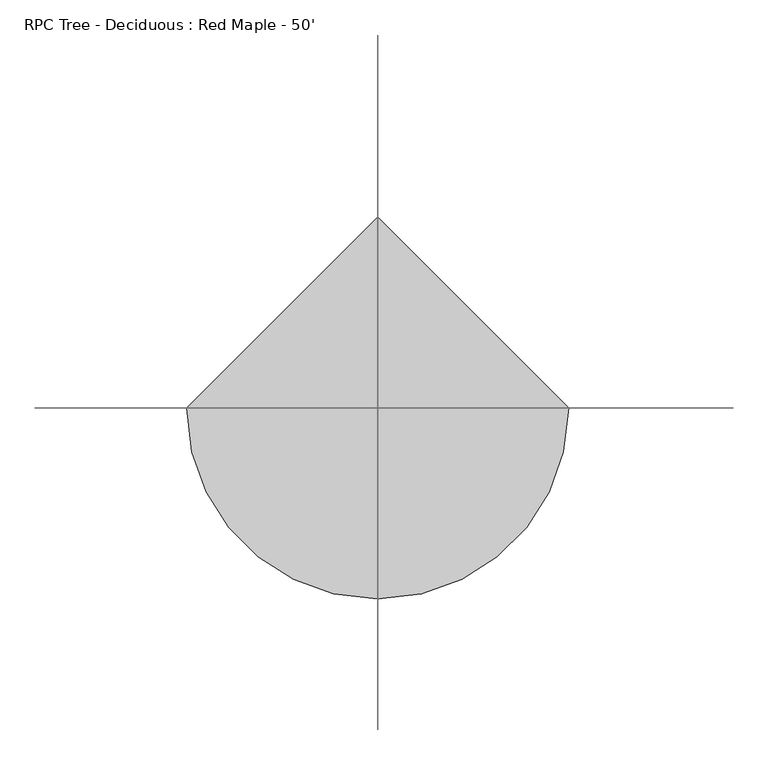
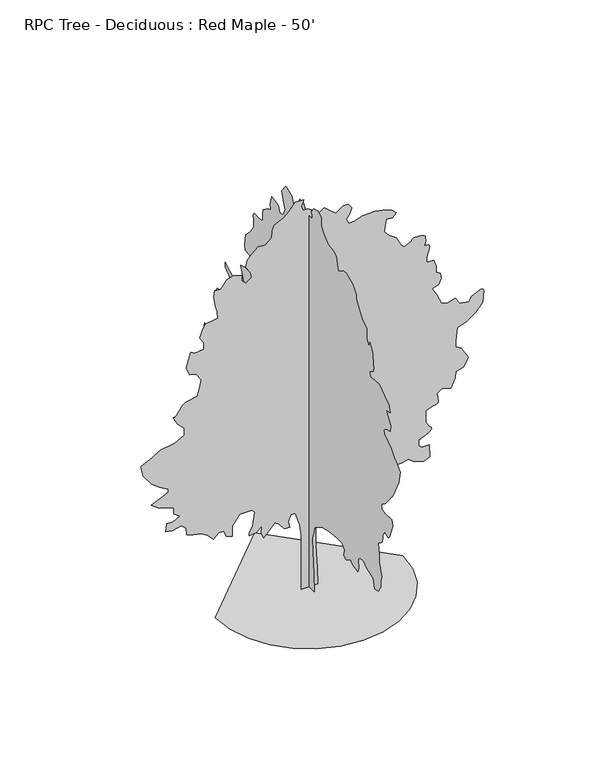
"""IFC4 building model written with IfcOpenShell, lengths in millimetres: geographic element geometry, RPC Tree - Deciduous : Red Maple - 50'."""

from ifc_helpers import new_model, si_unit, origin, place, context, project, spatial, triangles, source, transform, mapped, element, save


def rpc_tree_deciduous_red_maple_50_4953aeca(model_context):
    return source(origin(), model_context, "Body", "Tessellation", [
        triangles([(9.8e-06, 334.206708, 0.0219331), (9.8e-06, -334.2371567, 0.0219331), (9.8e-06, -289.6745243, 668.4650116), (9.8e-06, -245.1106201, 1537.4462723), (9.8e-06, -222.8301487, 2027.6369911), (9.8e-06, -289.6745243, 2272.7345306), (9.8e-06, -378.801079, 2562.392141), (9.8e-06, -534.7720456, 2651.5207123), (9.8e-06, -891.2740133, 2852.0541115), (9.8e-06, -1270.0602676, 2941.1783226), (9.8e-06, -1782.5353821, 3008.022789), (9.8e-06, -2139.0373135, 3008.022789), (9.8e-06, -2295.0061363, 2829.7697159), (9.8e-06, -2228.1618153, 2584.6721764), (9.8e-06, -2406.4148884, 2517.82771), (9.8e-06, -2696.0767136, 2673.8007477), (9.8e-06, -2701.2708733, 2654.7001694), (9.8e-06, -2709.0009247, 2635.6033699), (9.8e-06, -2721.7983994, 2616.5068611), (9.8e-06, -2742.1988983, 2597.4059921), (9.8e-06, -2772.7295929, 2578.3094833), (9.8e-06, -2815.9266655, 2559.2086143), (9.8e-06, -2874.3254265, 2540.1121056), (9.8e-06, -2935.3237381, 2523.6104965), (9.8e-06, -2985.8020523, 2511.7867996), (9.8e-06, -3027.5047394, 2503.8663528), (9.8e-06, -3062.1924477, 2499.0573441), (9.8e-06, -3091.6185585, 2496.5891808), (9.8e-06, -3117.53936, 2495.6790619), (9.8e-06, -3141.7030014, 2495.5476746), (9.8e-06, -3186.2674324, 2651.5207123), (9.8e-06, -3163.987397, 2985.7427536), (9.8e-06, -3297.6760391, 3119.4313957), (9.8e-06, -3520.4894737, 3141.7117218), (9.8e-06, -3698.7425468, 2963.458358), (9.8e-06, -4122.0887993, 2829.7697159), (9.8e-06, -4233.5061264, 2495.5476746), (9.8e-06, -4434.0392349, 2517.82771), (9.8e-06, -4612.2626587, 2785.2096451), (9.8e-06, -4612.2626587, 3008.022789), (9.8e-06, -4656.8395889, 3186.2758621), (9.8e-06, -4500.8837013, 3698.7466164), (9.8e-06, -4500.8837013, 3988.4085869), (9.8e-06, -4456.3064804, 4434.0392349), (9.8e-06, -4461.4288422, 4434.2932892), (9.8e-06, -4468.7103745, 4436.1135269), (9.8e-06, -4480.2672272, 4441.0664223), (9.8e-06, -4498.2588615, 4450.6763008), (9.8e-06, -4524.8441574, 4466.5087646), (9.8e-06, -4562.139846, 4490.1733086), (9.8e-06, -4612.2626587, 4523.1509468), (9.8e-06, -4661.1154907, 4563.9603745), (9.8e-06, -4694.7704132, 4609.4264946), (9.8e-06, -4715.7676781, 4658.7871445), (9.8e-06, -4726.605098, 4711.280452), (9.8e-06, -4729.8647827, 4766.1021057), (9.8e-06, -4728.044545, 4822.4902336), (9.8e-06, -4723.6840553, 4879.6823822), (9.8e-06, -4857.3729881, 5102.4833176), (9.8e-06, -4909.7392685, 5069.7591522), (9.8e-06, -4961.1320618, 5041.099855), (9.8e-06, -5010.5348602, 5020.6528473), (9.8e-06, -5057.059346, 5012.4399765), (9.8e-06, -5099.6893021, 5020.6528473), (9.8e-06, -5137.40793, 5049.2702866), (9.8e-06, -5169.3274933, 5102.4833176), (9.8e-06, -5392.1278473, 5637.237886), (9.8e-06, -5325.2836716, 5860.0388214), (9.8e-06, -4901.950209, 5837.7715759), (9.8e-06, -4656.8395889, 5860.0388214), (9.8e-06, -4679.1071251, 6082.8816147), (9.8e-06, -4736.4687401, 6116.7057129), (9.8e-06, -4794.2538757, 6153.0703537), (9.8e-06, -4852.7584442, 6194.5143356), (9.8e-06, -4912.4484055, 6243.5787827), (9.8e-06, -4973.7051315, 6302.7612167), (9.8e-06, -5036.9512711, 6374.6010178), (9.8e-06, -5102.4833176, 6461.638147), (9.8e-06, -5163.485408, 6547.4055862), (9.8e-06, -5213.9468628, 6615.6049118), (9.8e-06, -5255.6454803, 6669.1987335), (9.8e-06, -5290.3584778, 6711.1089661), (9.8e-06, -5319.7805191, 6744.2133408), (9.8e-06, -5345.6882401, 6771.5186508), (9.8e-06, -5369.8606018, 6795.8601883), (9.8e-06, -5748.6595734, 7553.4581314), (9.8e-06, -5860.0388214, 8043.636351), (9.8e-06, -5614.9706406, 8311.0136353), (9.8e-06, -5503.5495346, 8333.2808807), (9.8e-06, -5258.4394958, 8645.2356766), (9.8e-06, -5102.4833176, 8756.6567825), (9.8e-06, -5040.8458008, 8785.4858368), (9.8e-06, -4981.705806, 8815.5002838), (9.8e-06, -4927.646315, 8847.8430771), (9.8e-06, -4881.2067078, 8883.6996094), (9.8e-06, -4844.9269455, 8924.2546921), (9.8e-06, -4821.2624016, 8970.6100021), (9.8e-06, -4812.7957672, 9024.0346481), (9.8e-06, -4824.5220863, 9076.1047256), (9.8e-06, -4857.245961, 9118.8614182), (9.8e-06, -4907.5376587, 9153.8284698), (9.8e-06, -4971.8424545, 9182.5307877), (9.8e-06, -5046.687886, 9206.5758316), (9.8e-06, -5128.5183563, 9227.4885086), (9.8e-06, -5213.8619843, 9246.8350021), (9.8e-06, -5236.171669, 9491.9450409), (9.8e-06, -5124.750563, 9670.1684647), (9.8e-06, -4946.4847, 9915.2785034), (9.8e-06, -5213.8619843, 9982.1232605), (9.8e-06, -5124.750563, 10249.5011261), (9.8e-06, -4835.105452, 10427.7669891), (9.8e-06, -4500.8837013, 10672.8345886), (9.8e-06, -4211.2176613, 10650.5673431), (9.8e-06, -3943.8400864, 10628.3000977), (9.8e-06, -3899.2756554, 10806.5229401), (9.8e-06, -4032.9642975, 10895.6779633), (9.8e-06, -4056.6753502, 10900.7997437), (9.8e-06, -4079.4126251, 10908.0806946), (9.8e-06, -4100.198275, 10919.6381287), (9.8e-06, -4118.0628822, 10937.6300537), (9.8e-06, -4132.0285995, 10964.2156403), (9.8e-06, -4141.1219398, 11001.5110382), (9.8e-06, -4144.3731949, 11051.6335602), (9.8e-06, -4142.4215698, 11114.1181183), (9.8e-06, -4136.9689957, 11185.9567566), (9.8e-06, -4128.5869492, 11265.6286377), (9.8e-06, -4117.8681267, 11351.4803741), (9.8e-06, -4105.3967949, 11442.0318237), (9.8e-06, -4091.7528603, 11535.7156403), (9.8e-06, -4077.5287285, 11630.9656403), (9.8e-06, -3899.2756554, 11942.9198547), (9.8e-06, -3832.431189, 11764.6539917), (9.8e-06, -3721.0225822, 11965.1871002), (9.8e-06, -3721.0225822, 12388.5217255), (9.8e-06, -3431.3649719, 12566.7875885), (9.8e-06, -3230.8318634, 12834.1642914), (9.8e-06, -3030.2987549, 13123.8094025), (9.8e-06, -3030.2987549, 13279.80802), (9.8e-06, -2807.4812508, 13547.1858856), (9.8e-06, -2406.4148884, 13747.7189941), (9.8e-06, -2183.6015991, 13703.1414825), (9.8e-06, -1893.9397739, 13502.608374), (9.8e-06, -1737.9709511, 13992.7865936), (9.8e-06, -1581.9979134, 14104.2076996), (9.8e-06, -1225.495982, 14148.7852112), (9.8e-06, -958.1184071, 14416.1630768), (9.8e-06, -779.8695488, 14616.6961853), (9.8e-06, -779.8695488, 14928.6073792), (9.8e-06, -579.3363676, 15062.2968933), (9.8e-06, -311.9550138, 14995.4521362), (9.8e-06, -155.9861728, 14794.9190277), (9.8e-06, -179.3067879, 14742.7640717), (9.8e-06, -199.3143784, 14692.7264282), (9.8e-06, -212.6959562, 14647.0059631), (9.8e-06, -216.1389328, 14607.7211517), (9.8e-06, -206.3298659, 14576.9869812), (9.8e-06, -179.955749, 14556.9637848), (9.8e-06, -133.7040118, 14549.8514282), (9.8e-06, 178.2378669, 14549.8514282), (9.8e-06, 378.7710299, 14839.4965393), (9.8e-06, 601.58679, 14817.2292938), (9.8e-06, 712.9912909, 14549.8514282), (9.8e-06, 1002.653116, 14416.1630768), (9.8e-06, 1114.0575806, 14638.9634308), (9.8e-06, 1492.8439075, 14794.9190277), (9.8e-06, 1737.9413017, 14460.6975677), (9.8e-06, 1626.532695, 14081.9404541), (9.8e-06, 1537.4081932, 13836.829834), (9.8e-06, 1648.8169453, 13569.4531311), (9.8e-06, 1871.6300892, 13524.8756195), (9.8e-06, 1960.754591, 13769.9862396), (9.8e-06, 2406.385239, 13814.5625885), (9.8e-06, 2495.5139557, 13502.608374), (9.8e-06, 2450.9495247, 13279.80802), (9.8e-06, 2651.4826332, 13212.9632629), (9.8e-06, 2941.1402435, 12990.121051), (9.8e-06, 2963.4246391, 12834.1642914), (9.8e-06, 2963.4246391, 12566.7875885), (9.8e-06, 3074.8291763, 12499.9428314), (9.8e-06, 3342.2067513, 12499.9428314), (9.8e-06, 3394.3061874, 12508.8329865), (9.8e-06, 3443.8703133, 12513.8280304), (9.8e-06, 3488.3667252, 12511.0340149), (9.8e-06, 3525.264473, 12496.5558289), (9.8e-06, 3552.0276649, 12466.4995239), (9.8e-06, 3566.1247696, 12416.9269684), (9.8e-06, 3565.0239647, 12343.9860718), (9.8e-06, 3556.7733055, 12263.8491028), (9.8e-06, 3550.8634918, 12194.2952087), (9.8e-06, 3546.9012337, 12133.5047333), (9.8e-06, 3544.4967293, 12079.6998779), (9.8e-06, 3543.2604675, 12031.1853973), (9.8e-06, 3542.8075882, 11986.1427979), (9.8e-06, 3542.7439293, 11942.9198547), (9.8e-06, 3765.5573639, 11630.9656403), (9.8e-06, 4055.2149742, 11341.3205292), (9.8e-06, 4122.0591499, 10917.9452087), (9.8e-06, 4077.4990791, 10717.4121002), (9.8e-06, 3854.681575, 10695.143692), (9.8e-06, 3676.4328621, 10650.5673431), (9.8e-06, 3542.7439293, 10360.9222321), (9.8e-06, 3720.9929329, 10026.7007721), (9.8e-06, 4122.0591499, 10026.7007721), (9.8e-06, 4389.4198654, 9937.5457489), (9.8e-06, 4166.6235809, 9358.2566895), (9.8e-06, 4367.1526199, 9135.4138962), (9.8e-06, 4924.1750153, 9202.2580719), (9.8e-06, 5080.1736328, 9291.4119324), (9.8e-06, 5392.085408, 9447.3681107), (9.8e-06, 5369.8181625, 9291.4119324), (9.8e-06, 4968.7519455, 8934.8802063), (9.8e-06, 4812.7957672, 8444.7025681), (9.8e-06, 4991.019191, 8065.9035965), (9.8e-06, 5236.1298111, 8088.2132813), (9.8e-06, 5241.5056458, 8111.8350952), (9.8e-06, 5250.6074158, 8134.14478), (9.8e-06, 5267.1174545, 8153.7028885), (9.8e-06, 5294.7186768, 8169.1542709), (9.8e-06, 5337.1370178, 8179.1449402), (9.8e-06, 5398.0972504, 8182.3203278), (9.8e-06, 5481.2398499, 8177.3247025), (9.8e-06, 5882.3060669, 8132.7477722), (9.8e-06, 6082.8391754, 7843.1026611), (9.8e-06, 6015.9949997, 7531.1484467), (9.8e-06, 5770.8843796, 7352.9250229), (9.8e-06, 5570.3512711, 6862.704364), (9.8e-06, 5659.4632736, 6550.7920074), (9.8e-06, 5748.6171341, 6439.3709015), (9.8e-06, 5971.4174881, 6060.5719299), (9.8e-06, 6417.0612167, 6105.1488602), (9.8e-06, 6706.7057465, 6283.4147232), (9.8e-06, 6795.817749, 5882.3485062), (9.8e-06, 6372.4842865, 5681.8153976), (9.8e-06, 6082.8391754, 5592.6609558), (9.8e-06, 5882.3060669, 5147.0602478), (9.8e-06, 5770.8843796, 4879.6823822), (9.8e-06, 5637.1960281, 4500.8837013), (9.8e-06, 5392.085408, 4545.4606316), (9.8e-06, 5013.3288757, 4612.305098), (9.8e-06, 4701.3743706, 4545.4606316), (9.8e-06, 4478.5740166, 4188.9416954), (9.8e-06, 4768.218837, 3899.2840851), (9.8e-06, 5035.5961212, 3854.7196541), (9.8e-06, 5080.1736328, 3431.3690414), (9.8e-06, 5060.7422607, 3388.8198944), (9.8e-06, 5039.3639145, 3348.8063484), (9.8e-06, 5014.0910385, 3313.8558655), (9.8e-06, 4982.9760773, 3286.5086975), (9.8e-06, 4944.0714752, 3269.2957947), (9.8e-06, 4895.4308395, 3264.7492699), (9.8e-06, 4835.0633034, 3275.4003639), (9.8e-06, 4772.1133667, 3296.4484978), (9.8e-06, 4716.1911987, 3321.0019409), (9.8e-06, 4666.1108253, 3348.4804962), (9.8e-06, 4620.6871445, 3378.3001877), (9.8e-06, 4578.8193512, 3409.8680283), (9.8e-06, 4539.2377556, 3442.6087624), (9.8e-06, 4500.8412621, 3475.9334724), (9.8e-06, 4344.8850838, 3654.1865456), (9.8e-06, 4315.9714417, 3701.2825081), (9.8e-06, 4285.4913254, 3744.4795807), (9.8e-06, 4251.9209908, 3779.882943), (9.8e-06, 4213.6558846, 3803.593705), (9.8e-06, 4169.1551125, 3811.7132675), (9.8e-06, 4116.8649902, 3800.3468102), (9.8e-06, 4055.2149742, 3765.595443), (9.8e-06, 3977.9775375, 3720.4467453), (9.8e-06, 3882.0290337, 3679.9762505), (9.8e-06, 3770.4933998, 3643.4043549), (9.8e-06, 3646.482074, 3609.9482574), (9.8e-06, 3513.1192841, 3578.8332962), (9.8e-06, 3373.5205376, 3549.2760887), (9.8e-06, 3230.8022141, 3520.4979034), (9.8e-06, 2874.2960678, 3431.3690414), (9.8e-06, 2985.7046745, 3208.5558975), (9.8e-06, 3342.2067513, 2985.7427536), (9.8e-06, 3520.4598244, 2696.0807831), (9.8e-06, 3208.5178185, 2584.6721764), (9.8e-06, 3165.3844048, 2584.9980286), (9.8e-06, 3121.2772133, 2587.2714363), (9.8e-06, 3075.2186874, 2593.443734), (9.8e-06, 3026.2388283, 2605.4621864), (9.8e-06, 2973.3603699, 2625.2740585), (9.8e-06, 2915.6089531, 2654.831266), (9.8e-06, 2852.0157417, 2696.0807831), (9.8e-06, 2786.471196, 2744.4763756), (9.8e-06, 2723.2631355, 2794.0402107), (9.8e-06, 2662.0067001, 2844.5821838), (9.8e-06, 2602.3083092, 2895.8985283), (9.8e-06, 2543.7781609, 2947.8034996), (9.8e-06, 2486.0270348, 3000.097982), (9.8e-06, 2428.6652744, 3052.58722), (9.8e-06, 1983.0388412, 3186.2758621), (9.8e-06, 1626.532695, 3253.1203285), (9.8e-06, 1270.0306183, 3342.2448303), (9.8e-06, 913.5243994, 3275.4003639), (9.8e-06, 423.3332445, 3097.1472908), (9.8e-06, 289.6444752, 2918.8982872), (9.8e-06, 178.2378669, 2606.956572), (9.8e-06, 133.6735358, 2161.3257786), (9.8e-06, 178.2378669, 1559.7263077), (9.8e-06, 267.3623142, 690.7493345), (-3475.3367065, 0.0, 0.0), (-3383.4606285, -796.3160013, 0.0), (-3121.797821, -1527.6080647, 0.0), (-2711.2999123, -2172.9166409, 0.0), (-2172.9166409, -2711.2999123, 0.0), (-1527.6080647, -3121.797821, 0.0), (-796.3160013, -3383.4606285, 0.0), (0.0001519, -3475.3367065, 0.0), (796.3160013, -3383.4606285, 0.0), (1527.6080647, -3121.797821, 0.0), (2172.9166409, -2711.2999123, 0.0), (2711.2999123, -2172.9166409, 0.0), (3121.797821, -1527.6080647, 0.0), (3383.4606285, -796.3160013, 0.0), (3475.3367065, 0.0003046, 0.0), (-0.0004557, 3475.3367065, 0.0), (333.1458352, 0.0003808, 0.0087733), (-282.8415111, 0.0003808, 0.0087733), (-282.8415111, 0.0003199, 1140.7276096), (-282.8415111, 0.0002742, 1733.9027401), (-282.8415111, 0.0002589, 2121.744183), (-351.284808, 0.0002285, 2555.2207764), (-510.9849074, 0.000198, 3057.1337448), (-670.6875504, 0.000198, 3057.1337448), (-761.9455702, 0.0002132, 2806.1772606), (-716.3144165, 0.0002285, 2578.0342094), (-921.6439619, 0.0002285, 2600.8476425), (-1104.1600742, 0.0002132, 2828.9906937), (-1263.8626808, 0.0002132, 2943.0622192), (-1446.3745056, 0.0002132, 2737.7326012), (-1674.5175568, 0.0002285, 2509.5898407), (-1765.7755039, 0.0002285, 2714.9191681), (-1742.9620708, 0.0002132, 2988.6934456), (-1971.105122, 0.0002132, 2806.1772606), (-2222.0656757, 0.0002132, 2783.3638275), (-2222.0656757, 0.0002132, 2897.4353531), (-2085.1765022, 0.000198, 3125.5784042), (-2016.736203, 0.0001675, 3627.4954422), (-2130.8077286, 0.0001675, 3741.5669678), (-2564.2801071, 0.0001675, 3741.5669678), (-2838.0500244, 0.0001828, 3353.7214554), (-2838.0500244, 0.000198, 3194.0230637), (-2838.0500244, 0.0002132, 2965.8800125), (-3066.1974358, 0.000198, 3057.1337448), (-3157.4552376, 0.0001828, 3285.2808655), (-3339.9670624, 0.0001828, 3285.2808655), (-3545.2966805, 0.000198, 3102.7649712), (-3773.4397316, 0.0001828, 3330.9077316), (-4001.5868523, 0.0001828, 3467.7926903), (-4298.1914223, 0.0001675, 3536.2373497), (-4526.3260437, 0.0001675, 3627.4954422), (-4549.1435463, 0.0001523, 3878.4519264), (-4731.6428719, 0.0001371, 4038.1543877), (-5073.8658783, 0.0001523, 3969.7100189), (-5302.000209, 0.0001371, 4015.3409546), (-5279.1824158, 0.0001219, 4311.9074455), (-5028.2302917, 0.0001219, 4311.9074455), (-4800.095961, 0.0001219, 4448.8136238), (-5005.4124985, 0.0001066, 4608.4951561), (-5005.4124985, 9.14e-05, 4836.6719261), (-5233.5474106, 9.14e-05, 4927.9003693), (-5552.9523331, 9.14e-05, 5019.170961), (-5849.5400436, 7.62e-05, 5247.3052917), (-5484.4995346, 6.09e-05, 5407.0292633), (-5210.7296173, 6.09e-05, 5521.075209), (-5210.7296173, 4.57e-05, 5635.1635941), (-5552.9523331, 3.05e-05, 5840.4807129), (-5826.7222504, 3.05e-05, 6045.8396896), (-6146.1277542, 0.0, 6479.2911392), (-6237.3983459, -3.05e-05, 6889.9672348), (-6054.8990204, -3.05e-05, 6981.1953873), (-5803.9044571, -4.57e-05, 7095.2837723), (-5507.3173279, -4.57e-05, 7277.7830978), (-4982.5947052, -6.09e-05, 7369.0536896), (-4617.5544868, -6.09e-05, 7551.5530151), (-4617.5544868, -7.62e-05, 7825.3229324), (-4868.5487595, -9.14e-05, 8076.3174957), (-5028.2302917, -0.0001219, 8372.9052063), (-5013.3288757, -0.0001219, 8368.544426), (-4997.030452, -0.0001219, 8367.6130875), (-4977.9385941, -0.0001219, 8373.497612), (-4954.6551315, -0.0001219, 8389.4995422), (-4925.783638, -0.0001219, 8419.0907593), (-4889.969545, -0.0001219, 8465.6576843), (-4845.7312569, -0.0001219, 8532.5867386), (-4798.8259804, -0.0001219, 8603.4946198), (-4755.5187401, -0.0001371, 8661.2376068), (-4715.217421, -0.0001371, 8707.9737076), (-4677.2865967, -0.0001371, 8745.9463898), (-4641.1763008, -0.0001371, 8777.3578445), (-4606.2513977, -0.0001371, 8804.3666611), (-4571.9613396, -0.0001371, 8829.1738678), (-4138.4718109, -0.0001523, 8920.4450409), (-4047.2137184, -0.0001675, 9239.8499634), (-4001.5868523, -0.0001828, 9513.6198807), (-4184.1030373, -0.000198, 9787.389798), (-4412.2376587, -0.000198, 9855.8007385), (-4549.1435463, -0.0002285, 10152.3884491), (-4457.8729546, -0.0002437, 10471.7933716), (-4389.4198654, -0.0002589, 10722.7454956), (-4229.7299034, -0.0002437, 10631.5173431), (-3910.3287598, -0.0002589, 10677.1529297), (-3910.3287598, -0.0002742, 10928.1050537), (-4047.2137184, -0.0002742, 11156.2388031), (-3955.9559166, -0.0002894, 11407.1909271), (-3841.884391, -0.0003046, 11635.3258392), (-3385.5982887, -0.0003199, 11703.7786377), (-3408.4117218, -0.0003351, 11977.5491364), (-3476.8563812, -0.0003503, 12228.5012604), (-3522.4832474, -0.0003656, 12593.5417694), (-3499.6698143, -0.0003808, 12821.6766815), (-3271.5267632, -0.0003808, 12798.8583069), (-3157.4552376, -0.0003808, 12935.7650665), (-3043.3840027, -0.000396, 13095.4460175), (-2815.2365913, -0.000396, 13163.8988159), (-2495.8357384, -0.000396, 13072.6288055), (-2495.8357384, -0.0003808, 12867.3111053), (-2336.1372013, -0.0003808, 12707.6301544), (-2130.8077286, -0.0003808, 12867.3111053), (-2176.4345947, -0.000396, 13095.4460175), (-2336.1372013, -0.0004112, 13346.3981415), (-2290.5061203, -0.0004265, 13597.3932861), (-2107.9900806, -0.0004417, 13779.891449), (-1879.8470295, -0.0004569, 13985.2091492), (-1628.8905453, -0.0004417, 13962.3907745), (-1377.9342064, -0.0004569, 14167.7503326), (-1355.1164131, -0.0004722, 14418.7024567), (-1286.6761139, -0.0004874, 14624.0189941), (-944.457395, -0.0005026, 14783.7429657), (-739.1279222, -0.0005026, 14966.2422913), (-510.9849074, -0.0005179, 15240.0116272), (-191.5843088, -0.0005179, 15240.0116272), (-282.8415111, -0.0005026, 14989.0595032), (-214.3986139, -0.0005026, 14829.3366943), (-54.6980966, -0.0005026, 14829.3366943), (82.1881156, -0.0004874, 14738.1073792), (127.8167167, -0.0004874, 14555.5661957), (401.5887142, -0.0004874, 14532.7489838), (561.2896494, -0.0004874, 14646.8373688), (789.4326279, -0.0004722, 14464.3380432), (994.7621733, -0.0004722, 14281.7968597), (1268.5362328, -0.0004722, 14487.1552551), (1451.0524178, -0.0004722, 14487.1552551), (1587.9372311, -0.0004722, 14304.6140717), (1519.492717, -0.0004569, 14076.4791595), (1382.6077583, -0.0004417, 13916.7982086), (1473.8658508, -0.0004417, 13734.2570251), (1679.1953236, -0.0004417, 13734.2570251), (1998.5963219, -0.0004417, 13848.3454102), (2454.8824242, -0.0004417, 13848.3454102), (2728.656411, -0.0004417, 13802.7098236), (3070.8709877, -0.0004265, 13688.6214386), (3230.5734489, -0.0004265, 13528.939325), (3093.6844208, -0.0004112, 13369.2165161), (2865.5413696, -0.0004112, 13392.033728), (2819.9145035, -0.000396, 13186.7171906), (2797.0967102, -0.0003808, 12935.7650665), (2956.7994621, -0.0003808, 12730.4473663), (3230.5734489, -0.0003656, 12547.9061829), (3413.0852737, -0.0003351, 12182.8656738), (3527.1567993, -0.0003351, 12091.6375214), (3800.9310768, -0.0003503, 12228.5012604), (3806.3199921, -0.0003503, 12247.9326324), (3814.6976784, -0.0003503, 12266.5582397), (3829.0656967, -0.0003503, 12283.5769684), (3852.4125275, -0.0003503, 12298.2237488), (3887.7313019, -0.0003503, 12309.6544464), (3938.0148605, -0.0003503, 12317.1051544), (4006.2604042, -0.0003503, 12319.7724335), (4077.1647972, -0.0003503, 12317.1051544), (4134.8990639, -0.0003503, 12309.6544464), (4181.6604538, -0.0003503, 12298.2237488), (4219.6377869, -0.0003503, 12283.5769684), (4251.0320915, -0.0003503, 12266.5582397), (4278.0406174, -0.0003503, 12247.9326324), (4302.8481148, -0.0003503, 12228.5012604), (4325.6659081, -0.0003351, 12023.1847229), (4280.0303215, -0.0003199, 11863.5026093), (4333.1587646, -0.0003199, 11862.7410278), (4382.5194145, -0.0003199, 11857.6180847), (4424.3026199, -0.0003199, 11843.7328857), (4454.6978577, -0.0003199, 11816.6403534), (4469.9379158, -0.0003199, 11772.0209839), (4466.2125618, -0.0003199, 11705.4296997), (4439.7542931, -0.0003046, 11612.5086273), (4406.6071884, -0.0003046, 11514.2948547), (4384.2550644, -0.0003046, 11432.8033173), (4370.8779739, -0.0002894, 11365.2818573), (4364.6972466, -0.0002894, 11308.9352966), (4363.8929352, -0.0002894, 11261.0138031), (4366.6869507, -0.0002894, 11218.6384827), (4371.3012039, -0.0002894, 11179.0571777), (4622.2533279, -0.0002894, 11179.0571777), (4713.5242104, -0.0002589, 10905.2866791), (4713.5242104, -0.0002589, 10677.1529297), (4873.205452, -0.0002437, 10585.8817566), (4896.0232452, -0.0002285, 10380.5652191), (4804.7526535, -0.0002285, 10175.205661), (4576.6180321, -0.0002132, 10083.9775085), (4736.341713, -0.000198, 9787.389798), (4896.0232452, -0.0001828, 9422.3492889), (5124.157576, -0.0001675, 9308.2609039), (5420.7452866, -0.0001828, 9399.5314957), (5580.4692581, -0.0001675, 9148.5793716), (5922.6495346, -0.0001523, 9102.9437851), (6036.7379196, -0.0001675, 9262.6253174), (6128.9822891, -0.0001675, 9315.5418549), (6217.4594467, -0.0001675, 9362.9976791), (6298.3585785, -0.0001828, 9399.7431107), (6367.827594, -0.0001828, 9420.2749969), (6422.1835785, -0.0001828, 9419.3012192), (6457.5744415, -0.0001828, 9391.3610641), (6470.2318085, -0.0001675, 9331.0786972), (6468.87724, -0.0001675, 9255.5135422), (6465.151886, -0.0001675, 9184.7742554), (6459.4371185, -0.0001523, 9117.9725189), (6452.113147, -0.0001523, 9054.3874466), (6443.604364, -0.0001523, 8993.2155991), (6434.290979, -0.0001523, 8933.6105164), (6424.5962219, -0.0001523, 8874.8094543), (6173.6440979, -0.0001219, 8601.039537), (5854.2391754, -0.0001066, 8350.087413), (5489.1986664, -0.0001066, 8235.999028), (5443.5630798, -7.62e-05, 7734.09478), (5443.5630798, -6.09e-05, 7505.9174286), (5648.8796173, -6.09e-05, 7369.0536896), (5899.8741806, -3.05e-05, 6935.5603821), (5740.1507904, -1.52e-05, 6616.1973175), (5443.5630798, 0.0, 6524.9267258), (5420.7452866, 1.52e-05, 6296.7918137), (5261.0637543, 3.05e-05, 5931.7513046), (4941.6588318, 3.05e-05, 6045.8396896), (4743.9618874, 3.05e-05, 5894.7942581), (4742.4800011, 3.05e-05, 5897.2074829), (4741.8451561, 3.05e-05, 5895.8947723), (4742.9456703, 3.05e-05, 5887.1743744), (4746.6288757, 3.05e-05, 5867.2779144), (4753.7830902, 3.05e-05, 5832.5218964), (4765.2977943, 4.57e-05, 5779.2245682), (4781.9348602, 4.57e-05, 5703.6169739), (4792.1795837, 4.57e-05, 5626.9088654), (4785.6602142, 4.57e-05, 5570.562886), (4765.1707672, 6.09e-05, 5531.1931961), (4733.5476974, 6.09e-05, 5505.3697723), (4693.5004326, 6.09e-05, 5489.7486328), (4647.8651367, 6.09e-05, 5480.9009171), (4599.4355347, 6.09e-05, 5475.4402039), (4325.6659081, 6.09e-05, 5384.21147), (4325.6659081, 9.14e-05, 4927.9003693), (4462.5296471, 0.0001066, 4722.5835411), (4495.8883667, 0.0001066, 4693.1193512), (4523.828231, 0.0001066, 4662.8511406), (4540.9734055, 0.0001066, 4630.9740166), (4541.9468925, 0.0001066, 4596.7263977), (4521.4152969, 0.0001066, 4559.3036819), (4473.9173241, 0.0001219, 4517.8594093), (4394.1187065, 0.0001219, 4471.6311264), (4306.9545502, 0.0001219, 4428.7052582), (4239.0092789, 0.0001219, 4396.6165192), (4186.9775711, 0.0001219, 4373.4600838), (4147.7343269, 0.0001219, 4357.5005928), (4118.071312, 0.0001219, 4346.9172272), (4094.7922096, 0.0001219, 4339.9321884), (4074.7050636, 0.0001219, 4334.7252388), (4074.7050636, 0.0001371, 4106.5990471), (4188.7765892, 0.0001523, 3992.523452), (4462.5296471, 0.0001523, 3992.523452), (4485.3471497, 0.0001675, 3513.4239166), (4257.2128189, 0.0001828, 3422.1658241), (3915.0026024, 0.0001675, 3536.2373497), (3686.8595512, 0.0001675, 3695.9401016), (3458.7165001, 0.0001675, 3650.3088753), (3048.0575546, 0.0001675, 3627.4954422), (2797.0967102, 0.0001675, 3559.0507828), (2774.2832771, 0.000198, 3239.6499298), (2523.3267929, 0.000198, 3216.8364967), (2203.9259399, 0.000198, 3239.6499298), (2067.0367664, 0.000198, 3034.3203117), (1587.9372311, 0.0002132, 2965.8800125), (1222.9051517, 0.000198, 3057.1337448), (1222.9051517, 0.0002285, 2692.105735), (926.3218014, 0.0002285, 2714.9191681), (835.0637815, 0.0002132, 2897.4353531), (675.361175, 0.0002132, 2828.9906937), (492.8450626, 0.0002132, 2828.9906937), (424.4046907, 0.000198, 3034.3203117), (241.8881969, 0.0002132, 2828.9906937), (219.07391, 0.0002285, 2578.0342094), (241.8881969, 0.0002589, 2190.1886971), (241.8881969, 0.0002894, 1551.3867004), (310.3315301, 0.0003503, 638.810499)], [[130, 131, 132], [208, 209, 210], [208, 210, 211], [207, 208, 211], [230, 231, 232], [230, 232, 233], [276, 277, 278], [229, 230, 233], [229, 233, 234], [302, 1, 2], [302, 2, 3], [302, 3, 4], [301, 302, 4], [301, 4, 5], [300, 301, 5], [300, 5, 6], [299, 300, 6], [299, 6, 7], [108, 109, 110], [203, 204, 205], [206, 207, 211], [206, 211, 212], [108, 110, 111], [202, 203, 205], [13, 14, 15], [13, 15, 16], [236, 237, 238], [171, 172, 173], [170, 171, 173], [170, 173, 174], [36, 37, 38], [36, 38, 39], [36, 39, 40], [275, 276, 278], [275, 278, 279], [275, 279, 280], [275, 280, 281], [275, 281, 282], [275, 282, 283], [275, 283, 284], [275, 284, 285], [275, 285, 286], [275, 286, 287], [275, 287, 288], [275, 288, 289], [275, 289, 290], [274, 275, 290], [274, 290, 291], [274, 291, 292], [67, 68, 69], [66, 67, 69], [164, 165, 166], [164, 166, 167], [163, 164, 167], [163, 167, 168], [242, 243, 244], [29, 30, 31], [104, 105, 106], [197, 198, 199], [28, 29, 31], [298, 299, 7], [66, 69, 70], [65, 66, 70], [64, 65, 70], [63, 64, 70], [62, 63, 70], [61, 62, 70], [60, 61, 70], [59, 60, 70], [27, 28, 31], [150, 151, 152], [160, 161, 162], [159, 160, 162], [196, 197, 199], [195, 196, 199], [195, 199, 200], [26, 27, 31], [133, 134, 135], [242, 244, 245], [242, 245, 246], [242, 246, 247], [242, 247, 248], [242, 248, 249], [242, 249, 250], [242, 250, 251], [242, 251, 252], [242, 252, 253], [242, 253, 254], [242, 254, 255], [242, 255, 256], [242, 256, 257], [242, 257, 258], [242, 258, 259], [241, 242, 259], [241, 259, 260], [241, 260, 261], [241, 261, 262], [241, 262, 263], [241, 263, 264], [298, 7, 8], [274, 292, 293], [147, 148, 149], [147, 149, 150], [147, 150, 152], [147, 152, 153], [147, 153, 154], [147, 154, 155], [147, 155, 156], [36, 40, 41], [36, 41, 42], [35, 36, 42], [34, 35, 42], [34, 42, 43], [86, 87, 88], [86, 88, 89], [34, 43, 44], [104, 106, 107], [103, 104, 107], [102, 103, 107], [25, 26, 31], [25, 31, 32], [24, 25, 32], [23, 24, 32], [22, 23, 32], [21, 22, 32], [20, 21, 32], [19, 20, 32], [18, 19, 32], [17, 18, 32], [16, 17, 32], [13, 16, 32], [12, 13, 32], [102, 107, 108], [101, 102, 108], [129, 130, 132], [146, 147, 156], [100, 101, 108], [236, 238, 239], [146, 156, 157], [221, 222, 223], [221, 223, 224], [221, 224, 225], [220, 221, 225], [219, 220, 225], [218, 219, 225], [217, 218, 225], [216, 217, 225], [215, 216, 225], [214, 215, 225], [213, 214, 225], [213, 225, 226], [33, 34, 44], [235, 236, 239], [298, 8, 9], [297, 298, 9], [12, 32, 33], [58, 59, 70], [175, 176, 177], [85, 86, 89], [85, 89, 90], [85, 90, 91], [85, 91, 92], [84, 85, 92], [84, 92, 93], [83, 84, 93], [82, 83, 93], [82, 93, 94], [81, 82, 94], [80, 81, 94], [80, 94, 95], [79, 80, 95], [12, 33, 44], [78, 79, 95], [77, 78, 95], [76, 77, 95], [75, 76, 95], [74, 75, 95], [73, 74, 95], [72, 73, 95], [71, 72, 95], [71, 95, 96], [108, 111, 112], [108, 112, 113], [100, 108, 113], [100, 113, 114], [99, 100, 114], [98, 99, 114], [194, 195, 200], [128, 129, 132], [137, 138, 139], [175, 177, 178], [174, 175, 178], [241, 264, 265], [139, 140, 141], [139, 141, 142], [137, 139, 142], [229, 234, 235], [229, 235, 239], [228, 229, 239], [227, 228, 239], [227, 239, 240], [226, 227, 240], [213, 226, 240], [136, 137, 142], [142, 143, 144], [142, 144, 145], [145, 146, 157], [127, 128, 132], [11, 12, 44], [170, 174, 178], [194, 200, 201], [71, 96, 97], [145, 157, 158], [169, 170, 178], [212, 213, 240], [206, 212, 240], [205, 206, 240], [205, 240, 241], [205, 241, 265], [205, 265, 266], [205, 266, 267], [205, 267, 268], [205, 268, 269], [205, 269, 270], [205, 270, 271], [205, 271, 272], [205, 272, 273], [205, 273, 274], [205, 274, 293], [205, 293, 294], [205, 294, 295], [202, 205, 295], [202, 295, 296], [201, 202, 296], [201, 296, 297], [201, 297, 9], [201, 9, 10], [201, 10, 11], [201, 11, 44], [194, 201, 44], [193, 194, 44], [193, 44, 45], [193, 45, 46], [193, 46, 47], [193, 47, 48], [193, 48, 49], [193, 49, 50], [193, 50, 51], [193, 51, 52], [193, 52, 53], [193, 53, 54], [193, 54, 55], [193, 55, 56], [193, 56, 57], [193, 57, 58], [193, 58, 70], [193, 70, 71], [193, 71, 97], [193, 97, 98], [193, 98, 114], [193, 114, 115], [192, 193, 115], [191, 192, 115], [190, 191, 115], [189, 190, 115], [188, 189, 115], [187, 188, 115], [186, 187, 115], [185, 186, 115], [184, 185, 115], [183, 184, 115], [182, 183, 115], [181, 182, 115], [180, 181, 115], [179, 180, 115], [178, 179, 115], [169, 178, 115], [168, 169, 115], [163, 168, 115], [162, 163, 115], [159, 162, 115], [158, 159, 115], [145, 158, 115], [142, 145, 115], [136, 142, 115], [135, 136, 115], [133, 135, 115], [132, 133, 115], [127, 132, 115], [126, 127, 115], [126, 115, 116], [125, 126, 116], [124, 125, 116], [123, 124, 116], [122, 123, 116], [121, 122, 116], [121, 116, 117], [120, 121, 117], [120, 117, 118], [119, 120, 118], [317, 318, 303], [316, 317, 303], [316, 303, 304], [315, 316, 304], [315, 304, 305], [315, 305, 306], [314, 315, 306], [313, 314, 306], [313, 306, 307], [313, 307, 308], [313, 308, 309], [313, 309, 310], [313, 310, 311], [313, 311, 312], [379, 380, 381], [379, 381, 382], [364, 365, 366], [344, 345, 346], [332, 333, 334], [433, 434, 435], [327, 328, 329], [401, 402, 403], [327, 329, 330], [344, 346, 347], [343, 344, 347], [332, 334, 335], [432, 433, 435], [379, 382, 383], [534, 535, 536], [336, 337, 338], [336, 338, 339], [335, 336, 339], [582, 583, 584], [582, 584, 585], [593, 319, 320], [593, 320, 321], [592, 593, 321], [592, 321, 322], [591, 592, 322], [591, 322, 323], [412, 413, 414], [331, 332, 335], [591, 323, 324], [590, 591, 324], [568, 569, 570], [568, 570, 571], [568, 571, 572], [568, 572, 573], [567, 568, 573], [348, 349, 350], [532, 533, 534], [454, 455, 456], [454, 456, 457], [453, 454, 457], [357, 358, 359], [356, 357, 359], [355, 356, 359], [355, 359, 360], [363, 364, 366], [363, 366, 367], [589, 590, 324], [589, 324, 325], [576, 577, 578], [371, 372, 373], [335, 339, 340], [379, 383, 384], [504, 505, 506], [440, 441, 442], [417, 418, 419], [326, 327, 330], [494, 495, 496], [586, 587, 588], [362, 363, 367], [432, 435, 436], [588, 589, 325], [326, 330, 331], [352, 353, 354], [585, 586, 588], [452, 453, 457], [331, 335, 340], [379, 384, 385], [416, 417, 419], [415, 416, 419], [411, 412, 414], [531, 532, 534], [528, 529, 530], [528, 530, 531], [527, 528, 531], [431, 432, 436], [414, 415, 419], [411, 414, 419], [411, 419, 420], [410, 411, 420], [409, 410, 420], [576, 578, 579], [371, 373, 374], [370, 371, 374], [370, 374, 375], [369, 370, 375], [369, 375, 376], [368, 369, 376], [368, 376, 377], [407, 408, 409], [452, 457, 458], [451, 452, 458], [450, 451, 458], [450, 458, 459], [497, 498, 499], [497, 499, 500], [497, 500, 501], [445, 446, 447], [444, 445, 447], [443, 444, 447], [443, 447, 448], [326, 331, 340], [360, 361, 362], [494, 496, 497], [405, 406, 407], [405, 407, 409], [398, 399, 400], [398, 400, 401], [398, 401, 403], [398, 403, 404], [397, 398, 404], [579, 580, 581], [494, 497, 501], [425, 426, 427], [379, 385, 386], [429, 430, 431], [527, 531, 534], [477, 478, 479], [476, 477, 479], [475, 476, 479], [474, 475, 479], [473, 474, 479], [473, 479, 480], [472, 473, 480], [471, 472, 480], [470, 471, 480], [469, 470, 480], [468, 469, 480], [467, 468, 480], [466, 467, 480], [465, 466, 480], [464, 465, 480], [463, 464, 480], [566, 567, 573], [566, 573, 574], [566, 574, 575], [428, 429, 431], [428, 431, 436], [422, 423, 424], [422, 424, 425], [422, 425, 427], [421, 422, 427], [342, 343, 347], [437, 438, 439], [436, 437, 439], [428, 436, 439], [378, 379, 386], [378, 386, 387], [378, 387, 388], [378, 388, 389], [378, 389, 390], [378, 390, 391], [378, 391, 392], [378, 392, 393], [378, 393, 394], [378, 394, 395], [582, 585, 588], [351, 352, 354], [513, 514, 515], [512, 513, 515], [511, 512, 515], [511, 515, 516], [510, 511, 516], [510, 516, 517], [509, 510, 517], [509, 517, 518], [509, 518, 519], [508, 509, 519], [507, 508, 519], [507, 519, 520], [507, 520, 521], [507, 521, 522], [507, 522, 523], [507, 523, 524], [506, 507, 524], [506, 524, 525], [504, 506, 525], [503, 504, 525], [354, 355, 360], [579, 581, 582], [342, 347, 348], [342, 348, 350], [342, 350, 351], [342, 351, 354], [342, 354, 360], [342, 360, 362], [342, 362, 367], [342, 367, 368], [342, 368, 377], [341, 342, 377], [449, 450, 459], [527, 534, 536], [404, 405, 409], [341, 377, 378], [341, 378, 395], [341, 395, 396], [503, 525, 526], [440, 442, 443], [555, 556, 557], [554, 555, 557], [554, 557, 558], [553, 554, 558], [552, 553, 558], [552, 558, 559], [551, 552, 559], [551, 559, 560], [551, 560, 561], [551, 561, 562], [551, 562, 563], [551, 563, 564], [551, 564, 565], [551, 565, 566], [551, 566, 575], [550, 551, 575], [550, 575, 576], [460, 461, 462], [483, 484, 485], [482, 483, 485], [482, 485, 486], [481, 482, 486], [481, 486, 487], [480, 481, 487], [480, 487, 488], [463, 480, 488], [463, 488, 489], [463, 489, 490], [463, 490, 491], [463, 491, 492], [463, 492, 493], [463, 493, 494], [463, 494, 501], [341, 396, 397], [340, 341, 397], [326, 340, 397], [325, 326, 397], [588, 325, 397], [582, 588, 397], [579, 582, 397], [576, 579, 397], [550, 576, 397], [550, 397, 404], [550, 404, 409], [550, 409, 420], [550, 420, 421], [549, 550, 421], [549, 421, 427], [549, 427, 428], [549, 428, 439], [549, 439, 440], [549, 440, 443], [549, 443, 448], [549, 448, 449], [549, 449, 459], [549, 459, 460], [549, 460, 462], [549, 462, 463], [549, 463, 501], [549, 501, 502], [549, 502, 503], [548, 549, 503], [547, 548, 503], [526, 527, 536], [503, 526, 536], [544, 545, 546], [543, 544, 546], [543, 546, 547], [542, 543, 547], [541, 542, 547], [540, 541, 547], [503, 536, 537], [547, 503, 537], [547, 537, 538], [547, 538, 539], [540, 547, 539]], closed=False),
    ])


if __name__ == "__main__":
    model = new_model("IFC4")
    model_context = context("Model", 3, world=origin())
    ifc_project = project(units=[si_unit("LENGTHUNIT", "METRE", prefix="MILLI")], contexts=[model_context])
    site = spatial("IfcSite", under=ifc_project)
    building = spatial("IfcBuilding", under=site)
    placement = place(None, origin())
    rpc_tree_deciduous_red_maple_50_shape = rpc_tree_deciduous_red_maple_50_4953aeca(model_context)
    element("IfcGeographicElement", 1, ObjectType="RPC Tree - Deciduous : Red Maple - 50'", at=placement, inside=building, context=model_context, shape_type="MappedRepresentation", body=[
        mapped(rpc_tree_deciduous_red_maple_50_shape, transform((0.0, 0.0, 0.0), x_axis=(1.0, 0.0, 0.0), y_axis=(0.0, 1.0, 0.0), z_axis=(0.0, 0.0, 1.0))),
    ])
    save(model, "model.ifc")

# Revit data of these elements
# Type "RPC Tree - Deciduous : Red Maple - 50'"
#   COBie.Type.CreatedBy = "doug.wood@us.ibm.com"
#   COBie.Type.CreatedOn = "2016-04-14T02:07:24"
#   COBie.Type.Name = "Planting_RPC Tree - Deciduous_Red Maple - 50'"
#   COBie.Type.Category = "23-40 05 17 24 : Deciduous Trees"
#   COBie.Type.Description = "RPC Tree - Deciduous_Red Maple - 50'"
#   COBie.Type.Manufacturer = ""
#   COBie.Type.ModelNumber = ""
#   built-in parameter 1005198 = "{2, 15},{39, RPC-16-G0SR-83PX-Q347-6000-ST1L-LVER-AU},{1, 0},{1, 0},{2, 13},{1, 8},{5, Color},{1, 0},{1, 0},{3, 0.8},{3, 0.8},{3, 0.8},{1, 8},{7, BBoxMin},{1, 0},{1, 0},{1, 0},{1, 0},{1, 0},{1, 8},{7, BBoxMax},{1, 0},{1, 0},{1, 0},{1, 0},{1, 0},{2, 11},{9, RPCTypeId},{1, 0},{1, 0},{39, RPC-16-G0SR-83PX-Q347-6000-ST1L-LVER-AU},{1, 6},{14, RPCPlantHeight},{1, 0},{1, 0},{2, 30},{2, 11},{7, keyword},{1, 0},{1, 0},{34, :RPCs:Trees [General]:Geometry:RPC},{2, 11},{8, category},{1, 0},{1, 0},{15, Trees [General]},{2, 11},{12, LocalizedUID},{1, 0},{1, 0},{9, Red Maple},{2, 14},{6, Height},{1, 0},{1, 0},{2, 30},{1, 2},{16, Cast Reflections},{1, 0},{1, 0},{1, 0},{1, 2},{12, Cast Shadows},{1, 0},{1, 0},{1, 1},{1, 2},{9, Lock View},{1, 0},{1, 0},{1, 0},{1, 4},{5, ViewC},{1, 0},{1, 0},{1, 0},{21, assetlibrary_base.fbx},{1, 5},"
#   built-in parameter 1005195 = "RPC-16-G0SR-83PX-Q347-6000-ST1L-LVER-AU"
#   Type Comments = "Red Maple"
#   Assembly Code = "G2050500"
#   COBie.Type.ReplacementCost = 0
#   Height = 50' - 0"
#   COBie.Type = no
